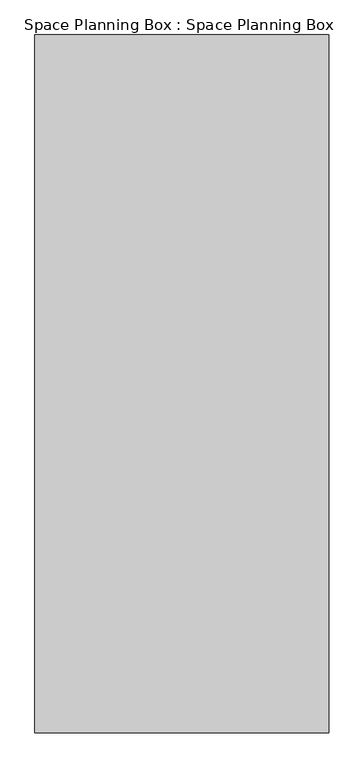
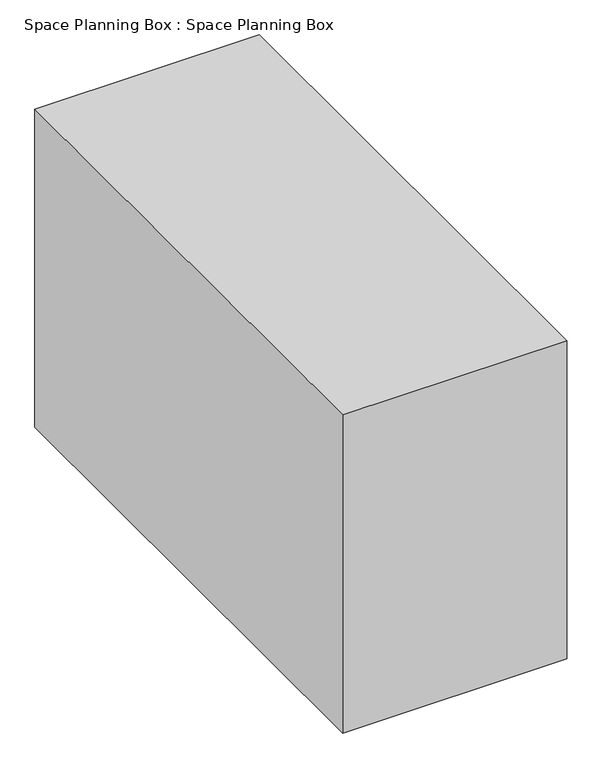
"""IFC4 building model written with IfcOpenShell, lengths in millimetres: proxy geometry, Space Planning Box : Space Planning Box."""

import ifcopenshell
import ifcopenshell.guid

model = None  # the IFC model being written
_history = None  # IfcOwnerHistory: only IFC2X3 demands one
_inside = {}  # id of a spatial element -> (the spatial element, [elements in it])
_under = {}  # id of a project, library or spatial element -> (it, [spatial elements below it])
_declared = {}  # id of a project -> (the project, [libraries it declares])
_typed = {}  # id of a type object -> (the type object, [elements of that type])
_made_of = {}  # id of a material, layer set ... -> (it, [elements and type objects made of it])


def new_model(schema):
    """Start an empty IFC model of exactly this schema.

    Asked for "IFC4X3", IfcOpenShell would pick the latest addendum, in which some entities
    have other attributes; the version numbers below select the first issue.
    IFC2X3 requires an IfcOwnerHistory on every rooted entity: one is made here for all.
    """
    global model, _history
    if schema == "IFC4X3":
        model = ifcopenshell.file(schema_version=(4, 3, 0, 0))
    else:
        model = ifcopenshell.file(schema=schema)
    _inside.clear()
    _under.clear()
    _declared.clear()
    _typed.clear()
    _made_of.clear()
    _history = None
    if model.schema == "IFC2X3":
        org = make("IfcOrganization", Name="unknown")
        user = make(
            "IfcPersonAndOrganization",
            ThePerson=make("IfcPerson", FamilyName="unknown"),
            TheOrganization=org,
        )
        app = make(
            "IfcApplication",
            ApplicationDeveloper=org,
            Version="unknown",
            ApplicationFullName="unknown",
            ApplicationIdentifier="unknown",
        )
        _history = make(
            "IfcOwnerHistory",
            OwningUser=user,
            OwningApplication=app,
            ChangeAction="ADDED",
            CreationDate=0,
        )
    return model


def make(cls, **values):
    """One entity of the class cls with the attributes given. An attribute that is None is left unset."""
    return model.create_entity(
        cls, **{name: value for name, value in values.items() if value is not None}
    )


def rooted(cls, **values):
    """An entity with a GlobalId (a new one), such as an element, a storey or a relation."""
    return make(cls, GlobalId=ifcopenshell.guid.new(), OwnerHistory=_history, **values)


def si_unit(unit_type, name, prefix=None):
    """IfcSIUnit, for example si_unit("LENGTHUNIT", "METRE", prefix="MILLI")."""
    return make("IfcSIUnit", UnitType=unit_type, Prefix=prefix, Name=name)


def assignment(units):
    """IfcUnitAssignment: the units of a project."""
    return None if units is None else make("IfcUnitAssignment", Units=units)


def point(xyz):
    """IfcCartesianPoint."""
    return None if xyz is None else make("IfcCartesianPoint", Coordinates=xyz)


def direction(xyz):
    """IfcDirection."""
    return None if xyz is None else make("IfcDirection", DirectionRatios=xyz)


def frame(location, z_axis=None, x_axis=None):
    """IfcAxis2Placement3D, a coordinate frame: its origin and axes. An axis left out is left unset."""
    return make(
        "IfcAxis2Placement3D",
        Location=point(location),
        Axis=direction(z_axis),
        RefDirection=direction(x_axis),
    )


def origin():
    """The frame at (0, 0, 0) with its axes left unset."""
    return frame((0.0, 0.0, 0.0))


def origin_with_axes():
    """The frame at (0, 0, 0) with the z axis (0, 0, 1) and the x axis (1, 0, 0) written out."""
    return frame((0.0, 0.0, 0.0), z_axis=(0.0, 0.0, 1.0), x_axis=(1.0, 0.0, 0.0))


def place(relative_to, where):
    """IfcLocalPlacement: puts the frame where relative to a parent placement (None: the world)."""
    return make(
        "IfcLocalPlacement", PlacementRelTo=relative_to, RelativePlacement=where
    )


def context(
    kind, dimensions, precision=None, world=None, true_north=None, identifier=None
):
    """IfcGeometricRepresentationContext, for example the 3D "Model" context."""
    return make(
        "IfcGeometricRepresentationContext",
        ContextIdentifier=identifier,
        ContextType=kind,
        CoordinateSpaceDimension=dimensions,
        Precision=precision,
        WorldCoordinateSystem=world,
        TrueNorth=true_north,
    )


def project(units=None, contexts=None):
    """IfcProject with its units and contexts."""
    return rooted(
        "IfcProject",
        Name="project",
        RepresentationContexts=contexts,
        UnitsInContext=assignment(units),
    )


def spatial(cls, under=None, at=None, **own):
    """A site, building, storey or space (cls), placed at a placement, below another one or the project."""
    s = rooted(cls, ObjectPlacement=at, **own)
    if under is not None:
        _under.setdefault(under.id(), (under, []))[1].append(s)
    return s


def polyline(points):
    """IfcPolyline through the points."""
    return make("IfcPolyline", Points=[point(p) for p in points])


def outline(outer, holes=None, kind="AREA"):
    """IfcArbitraryClosedProfileDef: a profile drawn as a closed curve; with holes, ...WithVoids."""
    if holes is None:
        return make("IfcArbitraryClosedProfileDef", ProfileType=kind, OuterCurve=outer)
    return make(
        "IfcArbitraryProfileDefWithVoids",
        ProfileType=kind,
        OuterCurve=outer,
        InnerCurves=holes,
    )


def extrude(swept, where, along, depth):
    """IfcExtrudedAreaSolid: the profile swept, set in the frame where, extruded along a direction by depth."""
    return make(
        "IfcExtrudedAreaSolid",
        SweptArea=swept,
        Position=where,
        ExtrudedDirection=direction(along),
        Depth=depth,
    )


def shape(context_of_items, identifier, shape_type, items):
    """IfcShapeRepresentation: the items that make up one representation, for example the "Body"."""
    return make(
        "IfcShapeRepresentation",
        ContextOfItems=context_of_items,
        RepresentationIdentifier=identifier,
        RepresentationType=shape_type,
        Items=items,
    )


def source(mapping_origin, context_of_items, identifier, shape_type, items):
    """IfcRepresentationMap: a shape defined once, which mapped items show again and again."""
    return make(
        "IfcRepresentationMap",
        MappingOrigin=mapping_origin,
        MappedRepresentation=shape(context_of_items, identifier, shape_type, items),
    )


def transform(
    local_origin,
    x_axis=None,
    y_axis=None,
    z_axis=None,
    scale=None,
    scale2=None,
    scale3=None,
    uniform=True,
):
    """IfcCartesianTransformationOperator3D, or its non-uniform kind. x_axis, y_axis, z_axis: its Axis1, 2, 3."""
    if uniform:
        return make(
            "IfcCartesianTransformationOperator3D",
            Axis1=direction(x_axis),
            Axis2=direction(y_axis),
            LocalOrigin=point(local_origin),
            Scale=scale,
            Axis3=direction(z_axis),
        )
    return make(
        "IfcCartesianTransformationOperator3DnonUniform",
        Axis1=direction(x_axis),
        Axis2=direction(y_axis),
        LocalOrigin=point(local_origin),
        Scale=scale,
        Axis3=direction(z_axis),
        Scale2=scale2,
        Scale3=scale3,
    )


def mapped(mapping_source, mapping_target):
    """IfcMappedItem: shows the shape of a source again, moved by a transform."""
    return make(
        "IfcMappedItem", MappingSource=mapping_source, MappingTarget=mapping_target
    )


def made_of(thing, what):
    """Note that an element or type object is made of a material, layer set ...; save() writes the relation."""
    if what is not None:
        _made_of.setdefault(what.id(), (what, []))[1].append(thing)
    return thing


def element(
    cls,
    number,
    at=None,
    inside=None,
    cuts=None,
    type_object=None,
    material=None,
    context=None,
    identifier="Body",
    shape_type=None,
    held_by="IfcProductDefinitionShape",
    body=None,
    shapes=None,
    **own,
):
    """One element of the class cls, such as IfcWall. Its Tag is "e" and its number.

    at: its placement. inside: the storey or other place that contains it. cuts: it is an
    opening in that element (IfcRelVoidsElement). A single representation is given by context,
    identifier, shape_type and body (its items); several are given by shapes. held_by: the class
    of the entity that holds the representations. save() writes the other relations.
    """
    e = rooted(cls, Tag="e%d" % number, ObjectPlacement=at, **own)
    if body is not None:
        shapes = [shape(context, identifier, shape_type, body)]
    if shapes is not None:
        e.Representation = make(held_by, Representations=shapes)
    if inside is not None:
        _inside.setdefault(inside.id(), (inside, []))[1].append(e)
    if cuts is not None:
        rooted(
            "IfcRelVoidsElement", RelatingBuildingElement=cuts, RelatedOpeningElement=e
        )
    if type_object is not None:
        _typed.setdefault(type_object.id(), (type_object, []))[1].append(e)
    return made_of(e, material)


def aggregate(whole, parts):
    """IfcRelAggregates: a whole, such as a stair, and the parts it consists of."""
    return rooted("IfcRelAggregates", RelatingObject=whole, RelatedObjects=parts)


def save(model, path):
    """Write the relations noted so far, then the file.

    IfcRelAggregates (storeys below a building ...), IfcRelContainedInSpatialStructure (elements
    in a storey), IfcRelDefinesByType, IfcRelAssociatesMaterial and IfcRelDeclares: one each for
    every whole, place, type object, material and project.
    """
    for whole, parts in _under.values():
        aggregate(whole, parts)
    for where, things in _inside.values():
        rooted(
            "IfcRelContainedInSpatialStructure",
            RelatedElements=things,
            RelatingStructure=where,
        )
    for kind, things in _typed.values():
        rooted("IfcRelDefinesByType", RelatedObjects=things, RelatingType=kind)
    for what, things in _made_of.values():
        rooted("IfcRelAssociatesMaterial", RelatedObjects=things, RelatingMaterial=what)
    for by, libraries in _declared.values():
        rooted("IfcRelDeclares", RelatingContext=by, RelatedDefinitions=libraries)
    model.write(path)


def space_planning_box_space_planning_box_3a820573(model_context):
    return source(origin(), model_context, "Body", "SweptSolid", [
        extrude(outline(polyline([(2000.0, 4750.0), (2000.0, -4750.0), (-2000.0, -4750.0), (-2000.0, 4750.0), (2000.0, 4750.0)])), origin_with_axes(), (0.0, 0.0, 1.0), 6000.0),
    ])


if __name__ == "__main__":
    model = new_model("IFC4")
    model_context = context("Model", 3, world=origin())
    ifc_project = project(units=[si_unit("LENGTHUNIT", "METRE", prefix="MILLI")], contexts=[model_context])
    site = spatial("IfcSite", under=ifc_project)
    building = spatial("IfcBuilding", under=site)
    placement = place(None, origin())
    space_planning_box_space_planning_box_shape = space_planning_box_space_planning_box_3a820573(model_context)
    element("IfcBuildingElementProxy", 1, Name="Space Planning Box : Space Planning Box", ObjectType="Space Planning Box : Space Planning Box", at=placement, inside=building, context=model_context, shape_type="MappedRepresentation", body=[
        mapped(space_planning_box_space_planning_box_shape, transform((0.0, 0.0, 0.0), x_axis=(1.0, 0.0, 0.0), y_axis=(0.0, 1.0, 0.0), z_axis=(0.0, 0.0, 1.0))),
    ])
    save(model, "model.ifc")

# Revit data of these elements
# Type "Space Planning Box : Space Planning Box"
#   Type Comments = "..."
#   Room Name [instance default] = "?"
#   Assembly Code = "..."
#   Width [instance default] = 1524 mm
#   Program Area [instance default] = 0 m²
#   Length [instance default] = 1524 mm
#   Height [instance default] = 1524 mm
#   Area [instance default] = 2.32258 m²
#   Fill Color [instance default] = Cyan
#   Default Elevation = 0
# Element 1 (IfcBuildingElementProxy, "Space Planning Box : Space Planning Box")
#   Room Name = "Stairway"
#   Width = 4000 mm
#   Program Area = 38 m²
#   Length = 9500 mm
#   Height = 6000 mm
#   Area = 38 m²
#   Fill Color = Lavender
#   Materials on its faces: "Lavender"
# Materials
#   "Cyan": class "Generic", colour RGB 0 255 255, transparency 0.2, Cost = 0
#   "Lavender": class "Generic", colour RGB 186 85 211, transparency 0.2, Cost = 0
